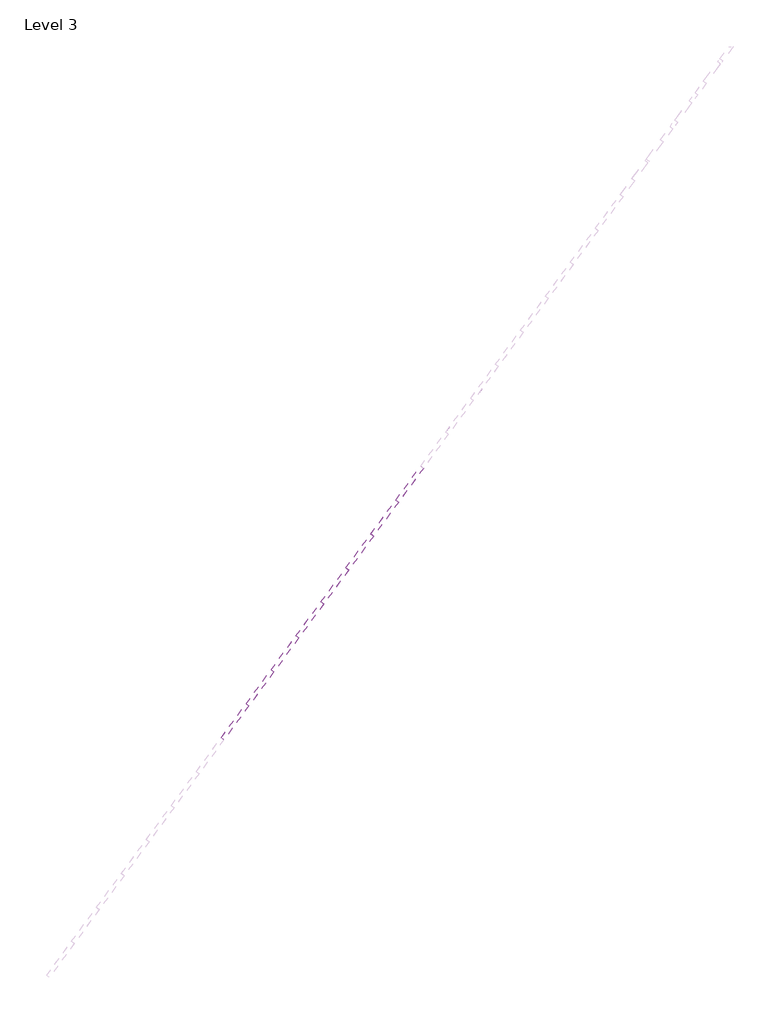
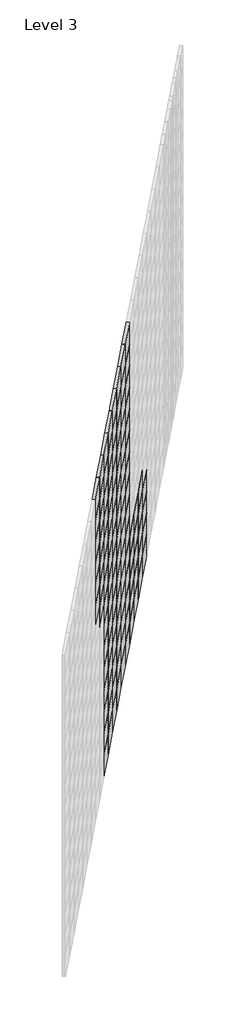
# One storey, part 2 of 9: 122 plates.
"""IFC4 building model written with IfcOpenShell, lengths in millimetres."""

import ifcopenshell
import ifcopenshell.guid

model = None  # the IFC model being written
_history = None  # IfcOwnerHistory: only IFC2X3 demands one
_inside = {}  # id of a spatial element -> (the spatial element, [elements in it])
_under = {}  # id of a project, library or spatial element -> (it, [spatial elements below it])
_declared = {}  # id of a project -> (the project, [libraries it declares])
_typed = {}  # id of a type object -> (the type object, [elements of that type])
_made_of = {}  # id of a material, layer set ... -> (it, [elements and type objects made of it])


def new_model(schema):
    """Start an empty IFC model of exactly this schema.

    Asked for "IFC4X3", IfcOpenShell would pick the latest addendum, in which some entities
    have other attributes; the version numbers below select the first issue.
    IFC2X3 requires an IfcOwnerHistory on every rooted entity: one is made here for all.
    """
    global model, _history
    if schema == "IFC4X3":
        model = ifcopenshell.file(schema_version=(4, 3, 0, 0))
    else:
        model = ifcopenshell.file(schema=schema)
    _inside.clear()
    _under.clear()
    _declared.clear()
    _typed.clear()
    _made_of.clear()
    _history = None
    if model.schema == "IFC2X3":
        org = make("IfcOrganization", Name="unknown")
        user = make(
            "IfcPersonAndOrganization",
            ThePerson=make("IfcPerson", FamilyName="unknown"),
            TheOrganization=org,
        )
        app = make(
            "IfcApplication",
            ApplicationDeveloper=org,
            Version="unknown",
            ApplicationFullName="unknown",
            ApplicationIdentifier="unknown",
        )
        _history = make(
            "IfcOwnerHistory",
            OwningUser=user,
            OwningApplication=app,
            ChangeAction="ADDED",
            CreationDate=0,
        )
    return model


def make(cls, **values):
    """One entity of the class cls with the attributes given. An attribute that is None is left unset."""
    return model.create_entity(
        cls, **{name: value for name, value in values.items() if value is not None}
    )


def rooted(cls, **values):
    """An entity with a GlobalId (a new one), such as an element, a storey or a relation."""
    return make(cls, GlobalId=ifcopenshell.guid.new(), OwnerHistory=_history, **values)


def si_unit(unit_type, name, prefix=None):
    """IfcSIUnit, for example si_unit("LENGTHUNIT", "METRE", prefix="MILLI")."""
    return make("IfcSIUnit", UnitType=unit_type, Prefix=prefix, Name=name)


def assignment(units):
    """IfcUnitAssignment: the units of a project."""
    return None if units is None else make("IfcUnitAssignment", Units=units)


def point(xyz):
    """IfcCartesianPoint."""
    return None if xyz is None else make("IfcCartesianPoint", Coordinates=xyz)


def direction(xyz):
    """IfcDirection."""
    return None if xyz is None else make("IfcDirection", DirectionRatios=xyz)


def frame(location, z_axis=None, x_axis=None):
    """IfcAxis2Placement3D, a coordinate frame: its origin and axes. An axis left out is left unset."""
    return make(
        "IfcAxis2Placement3D",
        Location=point(location),
        Axis=direction(z_axis),
        RefDirection=direction(x_axis),
    )


def origin():
    """The frame at (0, 0, 0) with its axes left unset."""
    return frame((0.0, 0.0, 0.0))


def origin_with_axes():
    """The frame at (0, 0, 0) with the z axis (0, 0, 1) and the x axis (1, 0, 0) written out."""
    return frame((0.0, 0.0, 0.0), z_axis=(0.0, 0.0, 1.0), x_axis=(1.0, 0.0, 0.0))


def place(relative_to, where):
    """IfcLocalPlacement: puts the frame where relative to a parent placement (None: the world)."""
    return make(
        "IfcLocalPlacement", PlacementRelTo=relative_to, RelativePlacement=where
    )


def context(
    kind, dimensions, precision=None, world=None, true_north=None, identifier=None
):
    """IfcGeometricRepresentationContext, for example the 3D "Model" context."""
    return make(
        "IfcGeometricRepresentationContext",
        ContextIdentifier=identifier,
        ContextType=kind,
        CoordinateSpaceDimension=dimensions,
        Precision=precision,
        WorldCoordinateSystem=world,
        TrueNorth=true_north,
    )


def project(units=None, contexts=None):
    """IfcProject with its units and contexts."""
    return rooted(
        "IfcProject",
        Name="project",
        RepresentationContexts=contexts,
        UnitsInContext=assignment(units),
    )


def spatial(cls, under=None, at=None, **own):
    """A site, building, storey or space (cls), placed at a placement, below another one or the project."""
    s = rooted(cls, ObjectPlacement=at, **own)
    if under is not None:
        _under.setdefault(under.id(), (under, []))[1].append(s)
    return s


def polyline(points):
    """IfcPolyline through the points."""
    return make("IfcPolyline", Points=[point(p) for p in points])


def outline(outer, holes=None, kind="AREA"):
    """IfcArbitraryClosedProfileDef: a profile drawn as a closed curve; with holes, ...WithVoids."""
    if holes is None:
        return make("IfcArbitraryClosedProfileDef", ProfileType=kind, OuterCurve=outer)
    return make(
        "IfcArbitraryProfileDefWithVoids",
        ProfileType=kind,
        OuterCurve=outer,
        InnerCurves=holes,
    )


def extrude(swept, where, along, depth):
    """IfcExtrudedAreaSolid: the profile swept, set in the frame where, extruded along a direction by depth."""
    return make(
        "IfcExtrudedAreaSolid",
        SweptArea=swept,
        Position=where,
        ExtrudedDirection=direction(along),
        Depth=depth,
    )


def shape(context_of_items, identifier, shape_type, items):
    """IfcShapeRepresentation: the items that make up one representation, for example the "Body"."""
    return make(
        "IfcShapeRepresentation",
        ContextOfItems=context_of_items,
        RepresentationIdentifier=identifier,
        RepresentationType=shape_type,
        Items=items,
    )


def source(mapping_origin, context_of_items, identifier, shape_type, items):
    """IfcRepresentationMap: a shape defined once, which mapped items show again and again."""
    return make(
        "IfcRepresentationMap",
        MappingOrigin=mapping_origin,
        MappedRepresentation=shape(context_of_items, identifier, shape_type, items),
    )


def transform(
    local_origin,
    x_axis=None,
    y_axis=None,
    z_axis=None,
    scale=None,
    scale2=None,
    scale3=None,
    uniform=True,
):
    """IfcCartesianTransformationOperator3D, or its non-uniform kind. x_axis, y_axis, z_axis: its Axis1, 2, 3."""
    if uniform:
        return make(
            "IfcCartesianTransformationOperator3D",
            Axis1=direction(x_axis),
            Axis2=direction(y_axis),
            LocalOrigin=point(local_origin),
            Scale=scale,
            Axis3=direction(z_axis),
        )
    return make(
        "IfcCartesianTransformationOperator3DnonUniform",
        Axis1=direction(x_axis),
        Axis2=direction(y_axis),
        LocalOrigin=point(local_origin),
        Scale=scale,
        Axis3=direction(z_axis),
        Scale2=scale2,
        Scale3=scale3,
    )


def mapped(mapping_source, mapping_target):
    """IfcMappedItem: shows the shape of a source again, moved by a transform."""
    return make(
        "IfcMappedItem", MappingSource=mapping_source, MappingTarget=mapping_target
    )


def made_of(thing, what):
    """Note that an element or type object is made of a material, layer set ...; save() writes the relation."""
    if what is not None:
        _made_of.setdefault(what.id(), (what, []))[1].append(thing)
    return thing


def element(
    cls,
    number,
    at=None,
    inside=None,
    cuts=None,
    type_object=None,
    material=None,
    context=None,
    identifier="Body",
    shape_type=None,
    held_by="IfcProductDefinitionShape",
    body=None,
    shapes=None,
    **own,
):
    """One element of the class cls, such as IfcWall. Its Tag is "e" and its number.

    at: its placement. inside: the storey or other place that contains it. cuts: it is an
    opening in that element (IfcRelVoidsElement). A single representation is given by context,
    identifier, shape_type and body (its items); several are given by shapes. held_by: the class
    of the entity that holds the representations. save() writes the other relations.
    """
    e = rooted(cls, Tag="e%d" % number, ObjectPlacement=at, **own)
    if body is not None:
        shapes = [shape(context, identifier, shape_type, body)]
    if shapes is not None:
        e.Representation = make(held_by, Representations=shapes)
    if inside is not None:
        _inside.setdefault(inside.id(), (inside, []))[1].append(e)
    if cuts is not None:
        rooted(
            "IfcRelVoidsElement", RelatingBuildingElement=cuts, RelatedOpeningElement=e
        )
    if type_object is not None:
        _typed.setdefault(type_object.id(), (type_object, []))[1].append(e)
    return made_of(e, material)


def aggregate(whole, parts):
    """IfcRelAggregates: a whole, such as a stair, and the parts it consists of."""
    return rooted("IfcRelAggregates", RelatingObject=whole, RelatedObjects=parts)


def save(model, path):
    """Write the relations noted so far, then the file.

    IfcRelAggregates (storeys below a building ...), IfcRelContainedInSpatialStructure (elements
    in a storey), IfcRelDefinesByType, IfcRelAssociatesMaterial and IfcRelDeclares: one each for
    every whole, place, type object, material and project.
    """
    for whole, parts in _under.values():
        aggregate(whole, parts)
    for where, things in _inside.values():
        rooted(
            "IfcRelContainedInSpatialStructure",
            RelatedElements=things,
            RelatingStructure=where,
        )
    for kind, things in _typed.values():
        rooted("IfcRelDefinesByType", RelatedObjects=things, RelatingType=kind)
    for what, things in _made_of.values():
        rooted("IfcRelAssociatesMaterial", RelatedObjects=things, RelatingMaterial=what)
    for by, libraries in _declared.values():
        rooted("IfcRelDeclares", RelatingContext=by, RelatedDefinitions=libraries)
    model.write(path)


def system_panel_glazed_2fc8f5ca(model_context):
    return source(origin(), model_context, "Body", "SweptSolid", [
        extrude(outline(polyline([(148.4832393, 24.5), (-148.4832393, 24.5), (-148.4832393, 49.5), (148.4832393, 49.5), (148.4832393, 24.5)])), origin_with_axes(), (0.0, 0.0, 1.0), 200.0),
    ])


model = new_model("IFC4")

# Units and contexts
model_context = context("Model", 3, world=origin())
ifc_project = project(units=[si_unit("LENGTHUNIT", "METRE", prefix="MILLI")], contexts=[model_context])

# Site, building, storey
site = spatial("IfcSite", under=ifc_project)
building = spatial("IfcBuilding", under=site)
storey = spatial("IfcBuildingStorey", under=building, Name="Level 3", Elevation=22950.0)

# Plates
placement = place(None, origin())
system_panel_glazed_shape = system_panel_glazed_2fc8f5ca(model_context)
element("IfcPlate", 1, ObjectType="System Panel : Glazed", at=placement, inside=storey, context=model_context, shape_type="MappedRepresentation", body=[
    mapped(system_panel_glazed_shape, transform((-35833.979291, 24676.4914868, 35100.0), x_axis=(0.5920548138930122, 0.8058976965757569, 0.0), y_axis=(-0.8058976965757569, 0.5920548138930122, 0.0), z_axis=(0.0, 0.0, 1.0))),
])
element("IfcPlate", 2, ObjectType="System Panel : Glazed", at=placement, inside=storey, context=model_context, shape_type="MappedRepresentation", body=[
    mapped(system_panel_glazed_shape, transform((-35658.1588579, 24915.8160876, 35100.0), x_axis=(0.5920548138930122, 0.8058976965757569, 0.0), y_axis=(-0.8058976965757569, 0.5920548138930122, 0.0), z_axis=(0.0, 0.0, 1.0))),
])
element("IfcPlate", 3, ObjectType="System Panel : Glazed", at=placement, inside=storey, context=model_context, shape_type="MappedRepresentation", body=[
    mapped(system_panel_glazed_shape, transform((-35482.3384249, 25155.1406885, 35100.0), x_axis=(0.5920548138930122, 0.8058976965757569, 0.0), y_axis=(-0.8058976965757569, 0.5920548138930122, 0.0), z_axis=(0.0, 0.0, 1.0))),
])
element("IfcPlate", 4, ObjectType="System Panel : Glazed", at=placement, inside=storey, context=model_context, shape_type="MappedRepresentation", body=[
    mapped(system_panel_glazed_shape, transform((-35306.5179918, 25394.4652893, 35100.0), x_axis=(0.5920548138930122, 0.8058976965757569, 0.0), y_axis=(-0.8058976965757569, 0.5920548138930122, 0.0), z_axis=(0.0, 0.0, 1.0))),
])
element("IfcPlate", 5, ObjectType="System Panel : Glazed", at=placement, inside=storey, context=model_context, shape_type="MappedRepresentation", body=[
    mapped(system_panel_glazed_shape, transform((-35130.6975588, 25633.7898902, 35100.0), x_axis=(0.5920548138930122, 0.8058976965757569, 0.0), y_axis=(-0.8058976965757569, 0.5920548138930122, 0.0), z_axis=(0.0, 0.0, 1.0))),
])
element("IfcPlate", 6, ObjectType="System Panel : Glazed", at=placement, inside=storey, context=model_context, shape_type="MappedRepresentation", body=[
    mapped(system_panel_glazed_shape, transform((-34954.8771257, 25873.114491, 35100.0), x_axis=(0.5920548138930122, 0.8058976965757569, 0.0), y_axis=(-0.8058976965757569, 0.5920548138930122, 0.0), z_axis=(0.0, 0.0, 1.0))),
])
element("IfcPlate", 7, ObjectType="System Panel : Glazed", at=placement, inside=storey, context=model_context, shape_type="MappedRepresentation", body=[
    mapped(system_panel_glazed_shape, transform((-34779.0566927, 26112.4390918, 35100.0), x_axis=(0.5920548138930122, 0.8058976965757569, 0.0), y_axis=(-0.8058976965757569, 0.5920548138930122, 0.0), z_axis=(0.0, 0.0, 1.0))),
])
element("IfcPlate", 8, ObjectType="System Panel : Glazed", at=placement, inside=storey, context=model_context, shape_type="MappedRepresentation", body=[
    mapped(system_panel_glazed_shape, transform((-34603.2362596, 26351.7636927, 35100.0), x_axis=(0.5920548138930122, 0.8058976965757569, 0.0), y_axis=(-0.8058976965757569, 0.5920548138930122, 0.0), z_axis=(0.0, 0.0, 1.0))),
])
element("IfcPlate", 9, ObjectType="System Panel : Glazed", at=placement, inside=storey, context=model_context, shape_type="MappedRepresentation", body=[
    mapped(system_panel_glazed_shape, transform((-34427.4158266, 26591.0882935, 35100.0), x_axis=(0.5920548138930122, 0.8058976965757569, 0.0), y_axis=(-0.8058976965757569, 0.5920548138930122, 0.0), z_axis=(0.0, 0.0, 1.0))),
])
element("IfcPlate", 10, ObjectType="System Panel : Glazed", at=placement, inside=storey, context=model_context, shape_type="MappedRepresentation", body=[
    mapped(system_panel_glazed_shape, transform((-34251.5953935, 26830.4128944, 35100.0), x_axis=(0.5920548138930122, 0.8058976965757569, 0.0), y_axis=(-0.8058976965757569, 0.5920548138930122, 0.0), z_axis=(0.0, 0.0, 1.0))),
])
element("IfcPlate", 11, ObjectType="System Panel : Glazed", at=placement, inside=storey, context=model_context, shape_type="MappedRepresentation", body=[
    mapped(system_panel_glazed_shape, transform((-35833.979291, 24676.4914868, 35300.0), x_axis=(0.5920548138930122, 0.8058976965757569, 0.0), y_axis=(-0.8058976965757569, 0.5920548138930122, 0.0), z_axis=(0.0, 0.0, 1.0))),
])
element("IfcPlate", 12, ObjectType="System Panel : Glazed", at=placement, inside=storey, context=model_context, shape_type="MappedRepresentation", body=[
    mapped(system_panel_glazed_shape, transform((-35658.1588579, 24915.8160876, 35300.0), x_axis=(0.5920548138930122, 0.8058976965757569, 0.0), y_axis=(-0.8058976965757569, 0.5920548138930122, 0.0), z_axis=(0.0, 0.0, 1.0))),
])
element("IfcPlate", 13, ObjectType="System Panel : Glazed", at=placement, inside=storey, context=model_context, shape_type="MappedRepresentation", body=[
    mapped(system_panel_glazed_shape, transform((-35482.3384249, 25155.1406885, 35300.0), x_axis=(0.5920548138930122, 0.8058976965757569, 0.0), y_axis=(-0.8058976965757569, 0.5920548138930122, 0.0), z_axis=(0.0, 0.0, 1.0))),
])
element("IfcPlate", 14, ObjectType="System Panel : Glazed", at=placement, inside=storey, context=model_context, shape_type="MappedRepresentation", body=[
    mapped(system_panel_glazed_shape, transform((-35306.5179918, 25394.4652893, 35300.0), x_axis=(0.5920548138930122, 0.8058976965757569, 0.0), y_axis=(-0.8058976965757569, 0.5920548138930122, 0.0), z_axis=(0.0, 0.0, 1.0))),
])
element("IfcPlate", 15, ObjectType="System Panel : Glazed", at=placement, inside=storey, context=model_context, shape_type="MappedRepresentation", body=[
    mapped(system_panel_glazed_shape, transform((-35130.6975588, 25633.7898902, 35300.0), x_axis=(0.5920548138930122, 0.8058976965757569, 0.0), y_axis=(-0.8058976965757569, 0.5920548138930122, 0.0), z_axis=(0.0, 0.0, 1.0))),
])
element("IfcPlate", 16, ObjectType="System Panel : Glazed", at=placement, inside=storey, context=model_context, shape_type="MappedRepresentation", body=[
    mapped(system_panel_glazed_shape, transform((-34954.8771257, 25873.114491, 35300.0), x_axis=(0.5920548138930122, 0.8058976965757569, 0.0), y_axis=(-0.8058976965757569, 0.5920548138930122, 0.0), z_axis=(0.0, 0.0, 1.0))),
])
element("IfcPlate", 17, ObjectType="System Panel : Glazed", at=placement, inside=storey, context=model_context, shape_type="MappedRepresentation", body=[
    mapped(system_panel_glazed_shape, transform((-34779.0566927, 26112.4390918, 35300.0), x_axis=(0.5920548138930122, 0.8058976965757569, 0.0), y_axis=(-0.8058976965757569, 0.5920548138930122, 0.0), z_axis=(0.0, 0.0, 1.0))),
])
element("IfcPlate", 18, ObjectType="System Panel : Glazed", at=placement, inside=storey, context=model_context, shape_type="MappedRepresentation", body=[
    mapped(system_panel_glazed_shape, transform((-34603.2362596, 26351.7636927, 35300.0), x_axis=(0.5920548138930122, 0.8058976965757569, 0.0), y_axis=(-0.8058976965757569, 0.5920548138930122, 0.0), z_axis=(0.0, 0.0, 1.0))),
])
element("IfcPlate", 19, ObjectType="System Panel : Glazed", at=placement, inside=storey, context=model_context, shape_type="MappedRepresentation", body=[
    mapped(system_panel_glazed_shape, transform((-34427.4158266, 26591.0882935, 35300.0), x_axis=(0.5920548138930122, 0.8058976965757569, 0.0), y_axis=(-0.8058976965757569, 0.5920548138930122, 0.0), z_axis=(0.0, 0.0, 1.0))),
])
element("IfcPlate", 20, ObjectType="System Panel : Glazed", at=placement, inside=storey, context=model_context, shape_type="MappedRepresentation", body=[
    mapped(system_panel_glazed_shape, transform((-34251.5953935, 26830.4128944, 35300.0), x_axis=(0.5920548138930122, 0.8058976965757569, 0.0), y_axis=(-0.8058976965757569, 0.5920548138930122, 0.0), z_axis=(0.0, 0.0, 1.0))),
])
element("IfcPlate", 21, ObjectType="System Panel : Glazed", at=placement, inside=storey, context=model_context, shape_type="MappedRepresentation", body=[
    mapped(system_panel_glazed_shape, transform((-35833.979291, 24676.4914868, 35500.0), x_axis=(0.5920548138930122, 0.8058976965757569, 0.0), y_axis=(-0.8058976965757569, 0.5920548138930122, 0.0), z_axis=(0.0, 0.0, 1.0))),
])
element("IfcPlate", 22, ObjectType="System Panel : Glazed", at=placement, inside=storey, context=model_context, shape_type="MappedRepresentation", body=[
    mapped(system_panel_glazed_shape, transform((-35658.1588579, 24915.8160876, 35500.0), x_axis=(0.5920548138930122, 0.8058976965757569, 0.0), y_axis=(-0.8058976965757569, 0.5920548138930122, 0.0), z_axis=(0.0, 0.0, 1.0))),
])
element("IfcPlate", 23, ObjectType="System Panel : Glazed", at=placement, inside=storey, context=model_context, shape_type="MappedRepresentation", body=[
    mapped(system_panel_glazed_shape, transform((-35482.3384249, 25155.1406885, 35500.0), x_axis=(0.5920548138930122, 0.8058976965757569, 0.0), y_axis=(-0.8058976965757569, 0.5920548138930122, 0.0), z_axis=(0.0, 0.0, 1.0))),
])
element("IfcPlate", 24, ObjectType="System Panel : Glazed", at=placement, inside=storey, context=model_context, shape_type="MappedRepresentation", body=[
    mapped(system_panel_glazed_shape, transform((-35306.5179918, 25394.4652893, 35500.0), x_axis=(0.5920548138930122, 0.8058976965757569, 0.0), y_axis=(-0.8058976965757569, 0.5920548138930122, 0.0), z_axis=(0.0, 0.0, 1.0))),
])
element("IfcPlate", 25, ObjectType="System Panel : Glazed", at=placement, inside=storey, context=model_context, shape_type="MappedRepresentation", body=[
    mapped(system_panel_glazed_shape, transform((-35130.6975588, 25633.7898902, 35500.0), x_axis=(0.5920548138930122, 0.8058976965757569, 0.0), y_axis=(-0.8058976965757569, 0.5920548138930122, 0.0), z_axis=(0.0, 0.0, 1.0))),
])
element("IfcPlate", 26, ObjectType="System Panel : Glazed", at=placement, inside=storey, context=model_context, shape_type="MappedRepresentation", body=[
    mapped(system_panel_glazed_shape, transform((-34954.8771257, 25873.114491, 35500.0), x_axis=(0.5920548138930122, 0.8058976965757569, 0.0), y_axis=(-0.8058976965757569, 0.5920548138930122, 0.0), z_axis=(0.0, 0.0, 1.0))),
])
element("IfcPlate", 27, ObjectType="System Panel : Glazed", at=placement, inside=storey, context=model_context, shape_type="MappedRepresentation", body=[
    mapped(system_panel_glazed_shape, transform((-34779.0566927, 26112.4390918, 35500.0), x_axis=(0.5920548138930122, 0.8058976965757569, 0.0), y_axis=(-0.8058976965757569, 0.5920548138930122, 0.0), z_axis=(0.0, 0.0, 1.0))),
])
element("IfcPlate", 28, ObjectType="System Panel : Glazed", at=placement, inside=storey, context=model_context, shape_type="MappedRepresentation", body=[
    mapped(system_panel_glazed_shape, transform((-34603.2362596, 26351.7636927, 35500.0), x_axis=(0.5920548138930122, 0.8058976965757569, 0.0), y_axis=(-0.8058976965757569, 0.5920548138930122, 0.0), z_axis=(0.0, 0.0, 1.0))),
])
element("IfcPlate", 29, ObjectType="System Panel : Glazed", at=placement, inside=storey, context=model_context, shape_type="MappedRepresentation", body=[
    mapped(system_panel_glazed_shape, transform((-34427.4158266, 26591.0882935, 35500.0), x_axis=(0.5920548138930122, 0.8058976965757569, 0.0), y_axis=(-0.8058976965757569, 0.5920548138930122, 0.0), z_axis=(0.0, 0.0, 1.0))),
])
element("IfcPlate", 30, ObjectType="System Panel : Glazed", at=placement, inside=storey, context=model_context, shape_type="MappedRepresentation", body=[
    mapped(system_panel_glazed_shape, transform((-34251.5953935, 26830.4128944, 35500.0), x_axis=(0.5920548138930122, 0.8058976965757569, 0.0), y_axis=(-0.8058976965757569, 0.5920548138930122, 0.0), z_axis=(0.0, 0.0, 1.0))),
])
element("IfcPlate", 31, ObjectType="System Panel : Glazed", at=placement, inside=storey, context=model_context, shape_type="MappedRepresentation", body=[
    mapped(system_panel_glazed_shape, transform((-35833.979291, 24676.4914868, 35700.0), x_axis=(0.5920548138930122, 0.8058976965757569, 0.0), y_axis=(-0.8058976965757569, 0.5920548138930122, 0.0), z_axis=(0.0, 0.0, 1.0))),
])
element("IfcPlate", 32, ObjectType="System Panel : Glazed", at=placement, inside=storey, context=model_context, shape_type="MappedRepresentation", body=[
    mapped(system_panel_glazed_shape, transform((-35658.1588579, 24915.8160876, 35700.0), x_axis=(0.5920548138930122, 0.8058976965757569, 0.0), y_axis=(-0.8058976965757569, 0.5920548138930122, 0.0), z_axis=(0.0, 0.0, 1.0))),
])
element("IfcPlate", 33, ObjectType="System Panel : Glazed", at=placement, inside=storey, context=model_context, shape_type="MappedRepresentation", body=[
    mapped(system_panel_glazed_shape, transform((-35482.3384249, 25155.1406885, 35700.0), x_axis=(0.5920548138930122, 0.8058976965757569, 0.0), y_axis=(-0.8058976965757569, 0.5920548138930122, 0.0), z_axis=(0.0, 0.0, 1.0))),
])
element("IfcPlate", 34, ObjectType="System Panel : Glazed", at=placement, inside=storey, context=model_context, shape_type="MappedRepresentation", body=[
    mapped(system_panel_glazed_shape, transform((-35306.5179918, 25394.4652893, 35700.0), x_axis=(0.5920548138930122, 0.8058976965757569, 0.0), y_axis=(-0.8058976965757569, 0.5920548138930122, 0.0), z_axis=(0.0, 0.0, 1.0))),
])
element("IfcPlate", 35, ObjectType="System Panel : Glazed", at=placement, inside=storey, context=model_context, shape_type="MappedRepresentation", body=[
    mapped(system_panel_glazed_shape, transform((-35130.6975588, 25633.7898902, 35700.0), x_axis=(0.5920548138930122, 0.8058976965757569, 0.0), y_axis=(-0.8058976965757569, 0.5920548138930122, 0.0), z_axis=(0.0, 0.0, 1.0))),
])
element("IfcPlate", 36, ObjectType="System Panel : Glazed", at=placement, inside=storey, context=model_context, shape_type="MappedRepresentation", body=[
    mapped(system_panel_glazed_shape, transform((-34954.8771257, 25873.114491, 35700.0), x_axis=(0.5920548138930122, 0.8058976965757569, 0.0), y_axis=(-0.8058976965757569, 0.5920548138930122, 0.0), z_axis=(0.0, 0.0, 1.0))),
])
element("IfcPlate", 37, ObjectType="System Panel : Glazed", at=placement, inside=storey, context=model_context, shape_type="MappedRepresentation", body=[
    mapped(system_panel_glazed_shape, transform((-34779.0566927, 26112.4390918, 35700.0), x_axis=(0.5920548138930122, 0.8058976965757569, 0.0), y_axis=(-0.8058976965757569, 0.5920548138930122, 0.0), z_axis=(0.0, 0.0, 1.0))),
])
element("IfcPlate", 38, ObjectType="System Panel : Glazed", at=placement, inside=storey, context=model_context, shape_type="MappedRepresentation", body=[
    mapped(system_panel_glazed_shape, transform((-34603.2362596, 26351.7636927, 35700.0), x_axis=(0.5920548138930122, 0.8058976965757569, 0.0), y_axis=(-0.8058976965757569, 0.5920548138930122, 0.0), z_axis=(0.0, 0.0, 1.0))),
])
element("IfcPlate", 39, ObjectType="System Panel : Glazed", at=placement, inside=storey, context=model_context, shape_type="MappedRepresentation", body=[
    mapped(system_panel_glazed_shape, transform((-34427.4158266, 26591.0882935, 35700.0), x_axis=(0.5920548138930122, 0.8058976965757569, 0.0), y_axis=(-0.8058976965757569, 0.5920548138930122, 0.0), z_axis=(0.0, 0.0, 1.0))),
])
element("IfcPlate", 40, ObjectType="System Panel : Glazed", at=placement, inside=storey, context=model_context, shape_type="MappedRepresentation", body=[
    mapped(system_panel_glazed_shape, transform((-34251.5953935, 26830.4128944, 35700.0), x_axis=(0.5920548138930122, 0.8058976965757569, 0.0), y_axis=(-0.8058976965757569, 0.5920548138930122, 0.0), z_axis=(0.0, 0.0, 1.0))),
])
element("IfcPlate", 41, ObjectType="System Panel : Glazed", at=placement, inside=storey, context=model_context, shape_type="MappedRepresentation", body=[
    mapped(system_panel_glazed_shape, transform((-35833.979291, 24676.4914868, 35900.0), x_axis=(0.5920548138930122, 0.8058976965757569, 0.0), y_axis=(-0.8058976965757569, 0.5920548138930122, 0.0), z_axis=(0.0, 0.0, 1.0))),
])
element("IfcPlate", 42, ObjectType="System Panel : Glazed", at=placement, inside=storey, context=model_context, shape_type="MappedRepresentation", body=[
    mapped(system_panel_glazed_shape, transform((-35658.1588579, 24915.8160876, 35900.0), x_axis=(0.5920548138930122, 0.8058976965757569, 0.0), y_axis=(-0.8058976965757569, 0.5920548138930122, 0.0), z_axis=(0.0, 0.0, 1.0))),
])
element("IfcPlate", 43, ObjectType="System Panel : Glazed", at=placement, inside=storey, context=model_context, shape_type="MappedRepresentation", body=[
    mapped(system_panel_glazed_shape, transform((-35482.3384249, 25155.1406885, 35900.0), x_axis=(0.5920548138930122, 0.8058976965757569, 0.0), y_axis=(-0.8058976965757569, 0.5920548138930122, 0.0), z_axis=(0.0, 0.0, 1.0))),
])
element("IfcPlate", 44, ObjectType="System Panel : Glazed", at=placement, inside=storey, context=model_context, shape_type="MappedRepresentation", body=[
    mapped(system_panel_glazed_shape, transform((-35306.5179918, 25394.4652893, 35900.0), x_axis=(0.5920548138930122, 0.8058976965757569, 0.0), y_axis=(-0.8058976965757569, 0.5920548138930122, 0.0), z_axis=(0.0, 0.0, 1.0))),
])
element("IfcPlate", 45, ObjectType="System Panel : Glazed", at=placement, inside=storey, context=model_context, shape_type="MappedRepresentation", body=[
    mapped(system_panel_glazed_shape, transform((-35130.6975588, 25633.7898902, 35900.0), x_axis=(0.5920548138930122, 0.8058976965757569, 0.0), y_axis=(-0.8058976965757569, 0.5920548138930122, 0.0), z_axis=(0.0, 0.0, 1.0))),
])
element("IfcPlate", 46, ObjectType="System Panel : Glazed", at=placement, inside=storey, context=model_context, shape_type="MappedRepresentation", body=[
    mapped(system_panel_glazed_shape, transform((-34954.8771257, 25873.114491, 35900.0), x_axis=(0.5920548138930122, 0.8058976965757569, 0.0), y_axis=(-0.8058976965757569, 0.5920548138930122, 0.0), z_axis=(0.0, 0.0, 1.0))),
])
element("IfcPlate", 47, ObjectType="System Panel : Glazed", at=placement, inside=storey, context=model_context, shape_type="MappedRepresentation", body=[
    mapped(system_panel_glazed_shape, transform((-34779.0566927, 26112.4390918, 35900.0), x_axis=(0.5920548138930122, 0.8058976965757569, 0.0), y_axis=(-0.8058976965757569, 0.5920548138930122, 0.0), z_axis=(0.0, 0.0, 1.0))),
])
element("IfcPlate", 48, ObjectType="System Panel : Glazed", at=placement, inside=storey, context=model_context, shape_type="MappedRepresentation", body=[
    mapped(system_panel_glazed_shape, transform((-34603.2362596, 26351.7636927, 35900.0), x_axis=(0.5920548138930122, 0.8058976965757569, 0.0), y_axis=(-0.8058976965757569, 0.5920548138930122, 0.0), z_axis=(0.0, 0.0, 1.0))),
])
element("IfcPlate", 49, ObjectType="System Panel : Glazed", at=placement, inside=storey, context=model_context, shape_type="MappedRepresentation", body=[
    mapped(system_panel_glazed_shape, transform((-34427.4158266, 26591.0882935, 35900.0), x_axis=(0.5920548138930122, 0.8058976965757569, 0.0), y_axis=(-0.8058976965757569, 0.5920548138930122, 0.0), z_axis=(0.0, 0.0, 1.0))),
])
element("IfcPlate", 50, ObjectType="System Panel : Glazed", at=placement, inside=storey, context=model_context, shape_type="MappedRepresentation", body=[
    mapped(system_panel_glazed_shape, transform((-35833.979291, 24676.4914868, 36100.0), x_axis=(0.5920548138930122, 0.8058976965757569, 0.0), y_axis=(-0.8058976965757569, 0.5920548138930122, 0.0), z_axis=(0.0, 0.0, 1.0))),
])
element("IfcPlate", 51, ObjectType="System Panel : Glazed", at=placement, inside=storey, context=model_context, shape_type="MappedRepresentation", body=[
    mapped(system_panel_glazed_shape, transform((-35658.1588579, 24915.8160876, 36100.0), x_axis=(0.5920548138930122, 0.8058976965757569, 0.0), y_axis=(-0.8058976965757569, 0.5920548138930122, 0.0), z_axis=(0.0, 0.0, 1.0))),
])
element("IfcPlate", 52, ObjectType="System Panel : Glazed", at=placement, inside=storey, context=model_context, shape_type="MappedRepresentation", body=[
    mapped(system_panel_glazed_shape, transform((-35482.3384249, 25155.1406885, 36100.0), x_axis=(0.5920548138930122, 0.8058976965757569, 0.0), y_axis=(-0.8058976965757569, 0.5920548138930122, 0.0), z_axis=(0.0, 0.0, 1.0))),
])
element("IfcPlate", 53, ObjectType="System Panel : Glazed", at=placement, inside=storey, context=model_context, shape_type="MappedRepresentation", body=[
    mapped(system_panel_glazed_shape, transform((-35306.5179918, 25394.4652893, 36100.0), x_axis=(0.5920548138930122, 0.8058976965757569, 0.0), y_axis=(-0.8058976965757569, 0.5920548138930122, 0.0), z_axis=(0.0, 0.0, 1.0))),
])
element("IfcPlate", 54, ObjectType="System Panel : Glazed", at=placement, inside=storey, context=model_context, shape_type="MappedRepresentation", body=[
    mapped(system_panel_glazed_shape, transform((-35130.6975588, 25633.7898902, 36100.0), x_axis=(0.5920548138930122, 0.8058976965757569, 0.0), y_axis=(-0.8058976965757569, 0.5920548138930122, 0.0), z_axis=(0.0, 0.0, 1.0))),
])
element("IfcPlate", 55, ObjectType="System Panel : Glazed", at=placement, inside=storey, context=model_context, shape_type="MappedRepresentation", body=[
    mapped(system_panel_glazed_shape, transform((-34954.8771257, 25873.114491, 36100.0), x_axis=(0.5920548138930122, 0.8058976965757569, 0.0), y_axis=(-0.8058976965757569, 0.5920548138930122, 0.0), z_axis=(0.0, 0.0, 1.0))),
])
element("IfcPlate", 56, ObjectType="System Panel : Glazed", at=placement, inside=storey, context=model_context, shape_type="MappedRepresentation", body=[
    mapped(system_panel_glazed_shape, transform((-35833.979291, 24676.4914868, 36300.0), x_axis=(0.5920548138930122, 0.8058976965757569, 0.0), y_axis=(-0.8058976965757569, 0.5920548138930122, 0.0), z_axis=(0.0, 0.0, 1.0))),
])
element("IfcPlate", 57, ObjectType="System Panel : Glazed", at=placement, inside=storey, context=model_context, shape_type="MappedRepresentation", body=[
    mapped(system_panel_glazed_shape, transform((-35658.1588579, 24915.8160876, 36300.0), x_axis=(0.5920548138930122, 0.8058976965757569, 0.0), y_axis=(-0.8058976965757569, 0.5920548138930122, 0.0), z_axis=(0.0, 0.0, 1.0))),
])
element("IfcPlate", 58, ObjectType="System Panel : Glazed", at=placement, inside=storey, context=model_context, shape_type="MappedRepresentation", body=[
    mapped(system_panel_glazed_shape, transform((-35482.3384249, 25155.1406885, 36300.0), x_axis=(0.5920548138930122, 0.8058976965757569, 0.0), y_axis=(-0.8058976965757569, 0.5920548138930122, 0.0), z_axis=(0.0, 0.0, 1.0))),
])
element("IfcPlate", 59, ObjectType="System Panel : Glazed", at=placement, inside=storey, context=model_context, shape_type="MappedRepresentation", body=[
    mapped(system_panel_glazed_shape, transform((-35306.5179918, 25394.4652893, 36300.0), x_axis=(0.5920548138930122, 0.8058976965757569, 0.0), y_axis=(-0.8058976965757569, 0.5920548138930122, 0.0), z_axis=(0.0, 0.0, 1.0))),
])
element("IfcPlate", 60, ObjectType="System Panel : Glazed", at=placement, inside=storey, context=model_context, shape_type="MappedRepresentation", body=[
    mapped(system_panel_glazed_shape, transform((-35130.6975588, 25633.7898902, 36300.0), x_axis=(0.5920548138930122, 0.8058976965757569, 0.0), y_axis=(-0.8058976965757569, 0.5920548138930122, 0.0), z_axis=(0.0, 0.0, 1.0))),
])
element("IfcPlate", 61, ObjectType="System Panel : Glazed", at=placement, inside=storey, context=model_context, shape_type="MappedRepresentation", body=[
    mapped(system_panel_glazed_shape, transform((-34954.8771257, 25873.114491, 36300.0), x_axis=(0.5920548138930122, 0.8058976965757569, 0.0), y_axis=(-0.8058976965757569, 0.5920548138930122, 0.0), z_axis=(0.0, 0.0, 1.0))),
])
element("IfcPlate", 62, ObjectType="System Panel : Glazed", at=placement, inside=storey, context=model_context, shape_type="MappedRepresentation", body=[
    mapped(system_panel_glazed_shape, transform((-35833.979291, 24676.4914868, 36500.0), x_axis=(0.5920548138930122, 0.8058976965757569, 0.0), y_axis=(-0.8058976965757569, 0.5920548138930122, 0.0), z_axis=(0.0, 0.0, 1.0))),
])
element("IfcPlate", 63, ObjectType="System Panel : Glazed", at=placement, inside=storey, context=model_context, shape_type="MappedRepresentation", body=[
    mapped(system_panel_glazed_shape, transform((-35658.1588579, 24915.8160876, 36500.0), x_axis=(0.5920548138930122, 0.8058976965757569, 0.0), y_axis=(-0.8058976965757569, 0.5920548138930122, 0.0), z_axis=(0.0, 0.0, 1.0))),
])
element("IfcPlate", 64, ObjectType="System Panel : Glazed", at=placement, inside=storey, context=model_context, shape_type="MappedRepresentation", body=[
    mapped(system_panel_glazed_shape, transform((-35482.3384249, 25155.1406885, 36500.0), x_axis=(0.5920548138930122, 0.8058976965757569, 0.0), y_axis=(-0.8058976965757569, 0.5920548138930122, 0.0), z_axis=(0.0, 0.0, 1.0))),
])
element("IfcPlate", 65, ObjectType="System Panel : Glazed", at=placement, inside=storey, context=model_context, shape_type="MappedRepresentation", body=[
    mapped(system_panel_glazed_shape, transform((-35306.5179918, 25394.4652893, 36500.0), x_axis=(0.5920548138930122, 0.8058976965757569, 0.0), y_axis=(-0.8058976965757569, 0.5920548138930122, 0.0), z_axis=(0.0, 0.0, 1.0))),
])
element("IfcPlate", 66, ObjectType="System Panel : Glazed", at=placement, inside=storey, context=model_context, shape_type="MappedRepresentation", body=[
    mapped(system_panel_glazed_shape, transform((-35130.6975588, 25633.7898902, 36500.0), x_axis=(0.5920548138930122, 0.8058976965757569, 0.0), y_axis=(-0.8058976965757569, 0.5920548138930122, 0.0), z_axis=(0.0, 0.0, 1.0))),
])
element("IfcPlate", 67, ObjectType="System Panel : Glazed", at=placement, inside=storey, context=model_context, shape_type="MappedRepresentation", body=[
    mapped(system_panel_glazed_shape, transform((-34954.8771257, 25873.114491, 36500.0), x_axis=(0.5920548138930122, 0.8058976965757569, 0.0), y_axis=(-0.8058976965757569, 0.5920548138930122, 0.0), z_axis=(0.0, 0.0, 1.0))),
])
element("IfcPlate", 68, ObjectType="System Panel : Glazed", at=placement, inside=storey, context=model_context, shape_type="MappedRepresentation", body=[
    mapped(system_panel_glazed_shape, transform((-36009.7997241, 24437.166886, 36700.0), x_axis=(0.5920548138930122, 0.8058976965757569, 0.0), y_axis=(-0.8058976965757569, 0.5920548138930122, 0.0), z_axis=(0.0, 0.0, 1.0))),
])
element("IfcPlate", 69, ObjectType="System Panel : Glazed", at=placement, inside=storey, context=model_context, shape_type="MappedRepresentation", body=[
    mapped(system_panel_glazed_shape, transform((-35833.979291, 24676.4914868, 36700.0), x_axis=(0.5920548138930122, 0.8058976965757569, 0.0), y_axis=(-0.8058976965757569, 0.5920548138930122, 0.0), z_axis=(0.0, 0.0, 1.0))),
])
element("IfcPlate", 70, ObjectType="System Panel : Glazed", at=placement, inside=storey, context=model_context, shape_type="MappedRepresentation", body=[
    mapped(system_panel_glazed_shape, transform((-35658.1588579, 24915.8160876, 36700.0), x_axis=(0.5920548138930122, 0.8058976965757569, 0.0), y_axis=(-0.8058976965757569, 0.5920548138930122, 0.0), z_axis=(0.0, 0.0, 1.0))),
])
element("IfcPlate", 71, ObjectType="System Panel : Glazed", at=placement, inside=storey, context=model_context, shape_type="MappedRepresentation", body=[
    mapped(system_panel_glazed_shape, transform((-35482.3384249, 25155.1406885, 36700.0), x_axis=(0.5920548138930122, 0.8058976965757569, 0.0), y_axis=(-0.8058976965757569, 0.5920548138930122, 0.0), z_axis=(0.0, 0.0, 1.0))),
])
element("IfcPlate", 72, ObjectType="System Panel : Glazed", at=placement, inside=storey, context=model_context, shape_type="MappedRepresentation", body=[
    mapped(system_panel_glazed_shape, transform((-35306.5179918, 25394.4652893, 36700.0), x_axis=(0.5920548138930122, 0.8058976965757569, 0.0), y_axis=(-0.8058976965757569, 0.5920548138930122, 0.0), z_axis=(0.0, 0.0, 1.0))),
])
element("IfcPlate", 73, ObjectType="System Panel : Glazed", at=placement, inside=storey, context=model_context, shape_type="MappedRepresentation", body=[
    mapped(system_panel_glazed_shape, transform((-35130.6975588, 25633.7898902, 36700.0), x_axis=(0.5920548138930122, 0.8058976965757569, 0.0), y_axis=(-0.8058976965757569, 0.5920548138930122, 0.0), z_axis=(0.0, 0.0, 1.0))),
])
element("IfcPlate", 74, ObjectType="System Panel : Glazed", at=placement, inside=storey, context=model_context, shape_type="MappedRepresentation", body=[
    mapped(system_panel_glazed_shape, transform((-34954.8771257, 25873.114491, 36700.0), x_axis=(0.5920548138930122, 0.8058976965757569, 0.0), y_axis=(-0.8058976965757569, 0.5920548138930122, 0.0), z_axis=(0.0, 0.0, 1.0))),
])
element("IfcPlate", 75, ObjectType="System Panel : Glazed", at=placement, inside=storey, context=model_context, shape_type="MappedRepresentation", body=[
    mapped(system_panel_glazed_shape, transform((-36185.6201571, 24197.8422851, 36900.0), x_axis=(0.5920548138930122, 0.8058976965757569, 0.0), y_axis=(-0.8058976965757569, 0.5920548138930122, 0.0), z_axis=(0.0, 0.0, 1.0))),
])
element("IfcPlate", 76, ObjectType="System Panel : Glazed", at=placement, inside=storey, context=model_context, shape_type="MappedRepresentation", body=[
    mapped(system_panel_glazed_shape, transform((-36009.7997241, 24437.166886, 36900.0), x_axis=(0.5920548138930122, 0.8058976965757569, 0.0), y_axis=(-0.8058976965757569, 0.5920548138930122, 0.0), z_axis=(0.0, 0.0, 1.0))),
])
element("IfcPlate", 77, ObjectType="System Panel : Glazed", at=placement, inside=storey, context=model_context, shape_type="MappedRepresentation", body=[
    mapped(system_panel_glazed_shape, transform((-35833.979291, 24676.4914868, 36900.0), x_axis=(0.5920548138930122, 0.8058976965757569, 0.0), y_axis=(-0.8058976965757569, 0.5920548138930122, 0.0), z_axis=(0.0, 0.0, 1.0))),
])
element("IfcPlate", 78, ObjectType="System Panel : Glazed", at=placement, inside=storey, context=model_context, shape_type="MappedRepresentation", body=[
    mapped(system_panel_glazed_shape, transform((-35658.1588579, 24915.8160876, 36900.0), x_axis=(0.5920548138930122, 0.8058976965757569, 0.0), y_axis=(-0.8058976965757569, 0.5920548138930122, 0.0), z_axis=(0.0, 0.0, 1.0))),
])
element("IfcPlate", 79, ObjectType="System Panel : Glazed", at=placement, inside=storey, context=model_context, shape_type="MappedRepresentation", body=[
    mapped(system_panel_glazed_shape, transform((-35482.3384249, 25155.1406885, 36900.0), x_axis=(0.5920548138930122, 0.8058976965757569, 0.0), y_axis=(-0.8058976965757569, 0.5920548138930122, 0.0), z_axis=(0.0, 0.0, 1.0))),
])
element("IfcPlate", 80, ObjectType="System Panel : Glazed", at=placement, inside=storey, context=model_context, shape_type="MappedRepresentation", body=[
    mapped(system_panel_glazed_shape, transform((-35306.5179918, 25394.4652893, 36900.0), x_axis=(0.5920548138930122, 0.8058976965757569, 0.0), y_axis=(-0.8058976965757569, 0.5920548138930122, 0.0), z_axis=(0.0, 0.0, 1.0))),
])
element("IfcPlate", 81, ObjectType="System Panel : Glazed", at=placement, inside=storey, context=model_context, shape_type="MappedRepresentation", body=[
    mapped(system_panel_glazed_shape, transform((-35130.6975588, 25633.7898902, 36900.0), x_axis=(0.5920548138930122, 0.8058976965757569, 0.0), y_axis=(-0.8058976965757569, 0.5920548138930122, 0.0), z_axis=(0.0, 0.0, 1.0))),
])
element("IfcPlate", 82, ObjectType="System Panel : Glazed", at=placement, inside=storey, context=model_context, shape_type="MappedRepresentation", body=[
    mapped(system_panel_glazed_shape, transform((-34954.8771257, 25873.114491, 36900.0), x_axis=(0.5920548138930122, 0.8058976965757569, 0.0), y_axis=(-0.8058976965757569, 0.5920548138930122, 0.0), z_axis=(0.0, 0.0, 1.0))),
])
element("IfcPlate", 83, ObjectType="System Panel : Glazed", at=placement, inside=storey, context=model_context, shape_type="MappedRepresentation", body=[
    mapped(system_panel_glazed_shape, transform((-36185.6201571, 24197.8422851, 37100.0), x_axis=(0.5920548138930122, 0.8058976965757569, 0.0), y_axis=(-0.8058976965757569, 0.5920548138930122, 0.0), z_axis=(0.0, 0.0, 1.0))),
])
element("IfcPlate", 84, ObjectType="System Panel : Glazed", at=placement, inside=storey, context=model_context, shape_type="MappedRepresentation", body=[
    mapped(system_panel_glazed_shape, transform((-36009.7997241, 24437.166886, 37100.0), x_axis=(0.5920548138930122, 0.8058976965757569, 0.0), y_axis=(-0.8058976965757569, 0.5920548138930122, 0.0), z_axis=(0.0, 0.0, 1.0))),
])
element("IfcPlate", 85, ObjectType="System Panel : Glazed", at=placement, inside=storey, context=model_context, shape_type="MappedRepresentation", body=[
    mapped(system_panel_glazed_shape, transform((-35833.979291, 24676.4914868, 37100.0), x_axis=(0.5920548138930122, 0.8058976965757569, 0.0), y_axis=(-0.8058976965757569, 0.5920548138930122, 0.0), z_axis=(0.0, 0.0, 1.0))),
])
element("IfcPlate", 86, ObjectType="System Panel : Glazed", at=placement, inside=storey, context=model_context, shape_type="MappedRepresentation", body=[
    mapped(system_panel_glazed_shape, transform((-35658.1588579, 24915.8160876, 37100.0), x_axis=(0.5920548138930122, 0.8058976965757569, 0.0), y_axis=(-0.8058976965757569, 0.5920548138930122, 0.0), z_axis=(0.0, 0.0, 1.0))),
])
element("IfcPlate", 87, ObjectType="System Panel : Glazed", at=placement, inside=storey, context=model_context, shape_type="MappedRepresentation", body=[
    mapped(system_panel_glazed_shape, transform((-35482.3384249, 25155.1406885, 37100.0), x_axis=(0.5920548138930122, 0.8058976965757569, 0.0), y_axis=(-0.8058976965757569, 0.5920548138930122, 0.0), z_axis=(0.0, 0.0, 1.0))),
])
element("IfcPlate", 88, ObjectType="System Panel : Glazed", at=placement, inside=storey, context=model_context, shape_type="MappedRepresentation", body=[
    mapped(system_panel_glazed_shape, transform((-35306.5179918, 25394.4652893, 37100.0), x_axis=(0.5920548138930122, 0.8058976965757569, 0.0), y_axis=(-0.8058976965757569, 0.5920548138930122, 0.0), z_axis=(0.0, 0.0, 1.0))),
])
element("IfcPlate", 89, ObjectType="System Panel : Glazed", at=placement, inside=storey, context=model_context, shape_type="MappedRepresentation", body=[
    mapped(system_panel_glazed_shape, transform((-35130.6975588, 25633.7898902, 37100.0), x_axis=(0.5920548138930122, 0.8058976965757569, 0.0), y_axis=(-0.8058976965757569, 0.5920548138930122, 0.0), z_axis=(0.0, 0.0, 1.0))),
])
element("IfcPlate", 90, ObjectType="System Panel : Glazed", at=placement, inside=storey, context=model_context, shape_type="MappedRepresentation", body=[
    mapped(system_panel_glazed_shape, transform((-34954.8771257, 25873.114491, 37100.0), x_axis=(0.5920548138930122, 0.8058976965757569, 0.0), y_axis=(-0.8058976965757569, 0.5920548138930122, 0.0), z_axis=(0.0, 0.0, 1.0))),
])
element("IfcPlate", 91, ObjectType="System Panel : Glazed", at=placement, inside=storey, context=model_context, shape_type="MappedRepresentation", body=[
    mapped(system_panel_glazed_shape, transform((-36185.6201571, 24197.8422851, 37300.0), x_axis=(0.5920548138930122, 0.8058976965757569, 0.0), y_axis=(-0.8058976965757569, 0.5920548138930122, 0.0), z_axis=(0.0, 0.0, 1.0))),
])
element("IfcPlate", 92, ObjectType="System Panel : Glazed", at=placement, inside=storey, context=model_context, shape_type="MappedRepresentation", body=[
    mapped(system_panel_glazed_shape, transform((-36009.7997241, 24437.166886, 37300.0), x_axis=(0.5920548138930122, 0.8058976965757569, 0.0), y_axis=(-0.8058976965757569, 0.5920548138930122, 0.0), z_axis=(0.0, 0.0, 1.0))),
])
element("IfcPlate", 93, ObjectType="System Panel : Glazed", at=placement, inside=storey, context=model_context, shape_type="MappedRepresentation", body=[
    mapped(system_panel_glazed_shape, transform((-35833.979291, 24676.4914868, 37300.0), x_axis=(0.5920548138930122, 0.8058976965757569, 0.0), y_axis=(-0.8058976965757569, 0.5920548138930122, 0.0), z_axis=(0.0, 0.0, 1.0))),
])
element("IfcPlate", 94, ObjectType="System Panel : Glazed", at=placement, inside=storey, context=model_context, shape_type="MappedRepresentation", body=[
    mapped(system_panel_glazed_shape, transform((-35658.1588579, 24915.8160876, 37300.0), x_axis=(0.5920548138930122, 0.8058976965757569, 0.0), y_axis=(-0.8058976965757569, 0.5920548138930122, 0.0), z_axis=(0.0, 0.0, 1.0))),
])
element("IfcPlate", 95, ObjectType="System Panel : Glazed", at=placement, inside=storey, context=model_context, shape_type="MappedRepresentation", body=[
    mapped(system_panel_glazed_shape, transform((-35482.3384249, 25155.1406885, 37300.0), x_axis=(0.5920548138930122, 0.8058976965757569, 0.0), y_axis=(-0.8058976965757569, 0.5920548138930122, 0.0), z_axis=(0.0, 0.0, 1.0))),
])
element("IfcPlate", 96, ObjectType="System Panel : Glazed", at=placement, inside=storey, context=model_context, shape_type="MappedRepresentation", body=[
    mapped(system_panel_glazed_shape, transform((-35306.5179918, 25394.4652893, 37300.0), x_axis=(0.5920548138930122, 0.8058976965757569, 0.0), y_axis=(-0.8058976965757569, 0.5920548138930122, 0.0), z_axis=(0.0, 0.0, 1.0))),
])
element("IfcPlate", 97, ObjectType="System Panel : Glazed", at=placement, inside=storey, context=model_context, shape_type="MappedRepresentation", body=[
    mapped(system_panel_glazed_shape, transform((-35130.6975588, 25633.7898902, 37300.0), x_axis=(0.5920548138930122, 0.8058976965757569, 0.0), y_axis=(-0.8058976965757569, 0.5920548138930122, 0.0), z_axis=(0.0, 0.0, 1.0))),
])
element("IfcPlate", 98, ObjectType="System Panel : Glazed", at=placement, inside=storey, context=model_context, shape_type="MappedRepresentation", body=[
    mapped(system_panel_glazed_shape, transform((-34954.8771257, 25873.114491, 37300.0), x_axis=(0.5920548138930122, 0.8058976965757569, 0.0), y_axis=(-0.8058976965757569, 0.5920548138930122, 0.0), z_axis=(0.0, 0.0, 1.0))),
])
element("IfcPlate", 99, ObjectType="System Panel : Glazed", at=placement, inside=storey, context=model_context, shape_type="MappedRepresentation", body=[
    mapped(system_panel_glazed_shape, transform((-36185.6201571, 24197.8422851, 37500.0), x_axis=(0.5920548138930122, 0.8058976965757569, 0.0), y_axis=(-0.8058976965757569, 0.5920548138930122, 0.0), z_axis=(0.0, 0.0, 1.0))),
])
element("IfcPlate", 100, ObjectType="System Panel : Glazed", at=placement, inside=storey, context=model_context, shape_type="MappedRepresentation", body=[
    mapped(system_panel_glazed_shape, transform((-36009.7997241, 24437.166886, 37500.0), x_axis=(0.5920548138930122, 0.8058976965757569, 0.0), y_axis=(-0.8058976965757569, 0.5920548138930122, 0.0), z_axis=(0.0, 0.0, 1.0))),
])
element("IfcPlate", 101, ObjectType="System Panel : Glazed", at=placement, inside=storey, context=model_context, shape_type="MappedRepresentation", body=[
    mapped(system_panel_glazed_shape, transform((-35833.979291, 24676.4914868, 37500.0), x_axis=(0.5920548138930122, 0.8058976965757569, 0.0), y_axis=(-0.8058976965757569, 0.5920548138930122, 0.0), z_axis=(0.0, 0.0, 1.0))),
])
element("IfcPlate", 102, ObjectType="System Panel : Glazed", at=placement, inside=storey, context=model_context, shape_type="MappedRepresentation", body=[
    mapped(system_panel_glazed_shape, transform((-35658.1588579, 24915.8160876, 37500.0), x_axis=(0.5920548138930122, 0.8058976965757569, 0.0), y_axis=(-0.8058976965757569, 0.5920548138930122, 0.0), z_axis=(0.0, 0.0, 1.0))),
])
element("IfcPlate", 103, ObjectType="System Panel : Glazed", at=placement, inside=storey, context=model_context, shape_type="MappedRepresentation", body=[
    mapped(system_panel_glazed_shape, transform((-35482.3384249, 25155.1406885, 37500.0), x_axis=(0.5920548138930122, 0.8058976965757569, 0.0), y_axis=(-0.8058976965757569, 0.5920548138930122, 0.0), z_axis=(0.0, 0.0, 1.0))),
])
element("IfcPlate", 104, ObjectType="System Panel : Glazed", at=placement, inside=storey, context=model_context, shape_type="MappedRepresentation", body=[
    mapped(system_panel_glazed_shape, transform((-35306.5179918, 25394.4652893, 37500.0), x_axis=(0.5920548138930122, 0.8058976965757569, 0.0), y_axis=(-0.8058976965757569, 0.5920548138930122, 0.0), z_axis=(0.0, 0.0, 1.0))),
])
element("IfcPlate", 105, ObjectType="System Panel : Glazed", at=placement, inside=storey, context=model_context, shape_type="MappedRepresentation", body=[
    mapped(system_panel_glazed_shape, transform((-35130.6975588, 25633.7898902, 37500.0), x_axis=(0.5920548138930122, 0.8058976965757569, 0.0), y_axis=(-0.8058976965757569, 0.5920548138930122, 0.0), z_axis=(0.0, 0.0, 1.0))),
])
element("IfcPlate", 106, ObjectType="System Panel : Glazed", at=placement, inside=storey, context=model_context, shape_type="MappedRepresentation", body=[
    mapped(system_panel_glazed_shape, transform((-34954.8771257, 25873.114491, 37500.0), x_axis=(0.5920548138930122, 0.8058976965757569, 0.0), y_axis=(-0.8058976965757569, 0.5920548138930122, 0.0), z_axis=(0.0, 0.0, 1.0))),
])
element("IfcPlate", 107, ObjectType="System Panel : Glazed", at=placement, inside=storey, context=model_context, shape_type="MappedRepresentation", body=[
    mapped(system_panel_glazed_shape, transform((-36185.6201571, 24197.8422851, 37700.0), x_axis=(0.5920548138930122, 0.8058976965757569, 0.0), y_axis=(-0.8058976965757569, 0.5920548138930122, 0.0), z_axis=(0.0, 0.0, 1.0))),
])
element("IfcPlate", 108, ObjectType="System Panel : Glazed", at=placement, inside=storey, context=model_context, shape_type="MappedRepresentation", body=[
    mapped(system_panel_glazed_shape, transform((-36009.7997241, 24437.166886, 37700.0), x_axis=(0.5920548138930122, 0.8058976965757569, 0.0), y_axis=(-0.8058976965757569, 0.5920548138930122, 0.0), z_axis=(0.0, 0.0, 1.0))),
])
element("IfcPlate", 109, ObjectType="System Panel : Glazed", at=placement, inside=storey, context=model_context, shape_type="MappedRepresentation", body=[
    mapped(system_panel_glazed_shape, transform((-35833.979291, 24676.4914868, 37700.0), x_axis=(0.5920548138930122, 0.8058976965757569, 0.0), y_axis=(-0.8058976965757569, 0.5920548138930122, 0.0), z_axis=(0.0, 0.0, 1.0))),
])
element("IfcPlate", 110, ObjectType="System Panel : Glazed", at=placement, inside=storey, context=model_context, shape_type="MappedRepresentation", body=[
    mapped(system_panel_glazed_shape, transform((-35658.1588579, 24915.8160876, 37700.0), x_axis=(0.5920548138930122, 0.8058976965757569, 0.0), y_axis=(-0.8058976965757569, 0.5920548138930122, 0.0), z_axis=(0.0, 0.0, 1.0))),
])
element("IfcPlate", 111, ObjectType="System Panel : Glazed", at=placement, inside=storey, context=model_context, shape_type="MappedRepresentation", body=[
    mapped(system_panel_glazed_shape, transform((-35482.3384249, 25155.1406885, 37700.0), x_axis=(0.5920548138930122, 0.8058976965757569, 0.0), y_axis=(-0.8058976965757569, 0.5920548138930122, 0.0), z_axis=(0.0, 0.0, 1.0))),
])
element("IfcPlate", 112, ObjectType="System Panel : Glazed", at=placement, inside=storey, context=model_context, shape_type="MappedRepresentation", body=[
    mapped(system_panel_glazed_shape, transform((-35306.5179918, 25394.4652893, 37700.0), x_axis=(0.5920548138930122, 0.8058976965757569, 0.0), y_axis=(-0.8058976965757569, 0.5920548138930122, 0.0), z_axis=(0.0, 0.0, 1.0))),
])
element("IfcPlate", 113, ObjectType="System Panel : Glazed", at=placement, inside=storey, context=model_context, shape_type="MappedRepresentation", body=[
    mapped(system_panel_glazed_shape, transform((-35130.6975588, 25633.7898902, 37700.0), x_axis=(0.5920548138930122, 0.8058976965757569, 0.0), y_axis=(-0.8058976965757569, 0.5920548138930122, 0.0), z_axis=(0.0, 0.0, 1.0))),
])
element("IfcPlate", 114, ObjectType="System Panel : Glazed", at=placement, inside=storey, context=model_context, shape_type="MappedRepresentation", body=[
    mapped(system_panel_glazed_shape, transform((-34954.8771257, 25873.114491, 37700.0), x_axis=(0.5920548138930122, 0.8058976965757569, 0.0), y_axis=(-0.8058976965757569, 0.5920548138930122, 0.0), z_axis=(0.0, 0.0, 1.0))),
])
element("IfcPlate", 115, ObjectType="System Panel : Glazed", at=placement, inside=storey, context=model_context, shape_type="MappedRepresentation", body=[
    mapped(system_panel_glazed_shape, transform((-36185.6201571, 24197.8422851, 37900.0), x_axis=(0.5920548138930122, 0.8058976965757569, 0.0), y_axis=(-0.8058976965757569, 0.5920548138930122, 0.0), z_axis=(0.0, 0.0, 1.0))),
])
element("IfcPlate", 116, ObjectType="System Panel : Glazed", at=placement, inside=storey, context=model_context, shape_type="MappedRepresentation", body=[
    mapped(system_panel_glazed_shape, transform((-36009.7997241, 24437.166886, 37900.0), x_axis=(0.5920548138930122, 0.8058976965757569, 0.0), y_axis=(-0.8058976965757569, 0.5920548138930122, 0.0), z_axis=(0.0, 0.0, 1.0))),
])
element("IfcPlate", 117, ObjectType="System Panel : Glazed", at=placement, inside=storey, context=model_context, shape_type="MappedRepresentation", body=[
    mapped(system_panel_glazed_shape, transform((-35833.979291, 24676.4914868, 37900.0), x_axis=(0.5920548138930122, 0.8058976965757569, 0.0), y_axis=(-0.8058976965757569, 0.5920548138930122, 0.0), z_axis=(0.0, 0.0, 1.0))),
])
element("IfcPlate", 118, ObjectType="System Panel : Glazed", at=placement, inside=storey, context=model_context, shape_type="MappedRepresentation", body=[
    mapped(system_panel_glazed_shape, transform((-35658.1588579, 24915.8160876, 37900.0), x_axis=(0.5920548138930122, 0.8058976965757569, 0.0), y_axis=(-0.8058976965757569, 0.5920548138930122, 0.0), z_axis=(0.0, 0.0, 1.0))),
])
element("IfcPlate", 119, ObjectType="System Panel : Glazed", at=placement, inside=storey, context=model_context, shape_type="MappedRepresentation", body=[
    mapped(system_panel_glazed_shape, transform((-35482.3384249, 25155.1406885, 37900.0), x_axis=(0.5920548138930122, 0.8058976965757569, 0.0), y_axis=(-0.8058976965757569, 0.5920548138930122, 0.0), z_axis=(0.0, 0.0, 1.0))),
])
element("IfcPlate", 120, ObjectType="System Panel : Glazed", at=placement, inside=storey, context=model_context, shape_type="MappedRepresentation", body=[
    mapped(system_panel_glazed_shape, transform((-35306.5179918, 25394.4652893, 37900.0), x_axis=(0.5920548138930122, 0.8058976965757569, 0.0), y_axis=(-0.8058976965757569, 0.5920548138930122, 0.0), z_axis=(0.0, 0.0, 1.0))),
])
element("IfcPlate", 121, ObjectType="System Panel : Glazed", at=placement, inside=storey, context=model_context, shape_type="MappedRepresentation", body=[
    mapped(system_panel_glazed_shape, transform((-35130.6975588, 25633.7898902, 37900.0), x_axis=(0.5920548138930122, 0.8058976965757569, 0.0), y_axis=(-0.8058976965757569, 0.5920548138930122, 0.0), z_axis=(0.0, 0.0, 1.0))),
])
element("IfcPlate", 122, ObjectType="System Panel : Glazed", at=placement, inside=storey, context=model_context, shape_type="MappedRepresentation", body=[
    mapped(system_panel_glazed_shape, transform((-34954.8771257, 25873.114491, 37900.0), x_axis=(0.5920548138930122, 0.8058976965757569, 0.0), y_axis=(-0.8058976965757569, 0.5920548138930122, 0.0), z_axis=(0.0, 0.0, 1.0))),
])

save(model, "model.ifc")

# Revit data of these elements
# Elements 1, 2, 3, 4, 5, 6, 7, 8, 9, 10, 11, 12, 13, 14, 15, 16, 17, 18, 19, 20, 21, 22, 23, 24, 25, 26, 27, 28, 29, 30, 31, 32, 33, 34, 35, 36, 37, 38, 39, 40, 41, 42, 43, 44, 45, 46, 47, 48, 49, 50, 51, 52, 53, 54, 55, 56, 57, 58, 59, 60, 61, 62, 63, 64, 65, 66, 67, 68, 69, 70, 71, 72, 73, 74, 75, 76, 77, 78, 79, 80, 81, 82, 83, 84, 85, 86, 87, 88, 89, 90, 91, 92, 93, 94, 95, 96, 97, 98, 99, 100, 101, 102, 103, 104, 105, 106, 107, 108, 109, 110, 111, 112, 113, 114, 115, 116, 117, 118, 119, 120, 121, 122 (IfcPlate, "System Panel : Glazed")
#   Phase Created = New Construction
#   Materials on its faces: "Glass"
# Materials
#   "Glass": class "Glass", colour RGB 218 227 224, transparency 0.85, Description = "Soda Lime Glass", Cost = 0
